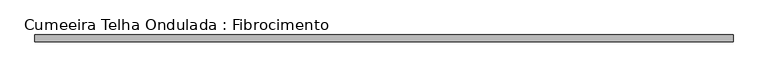
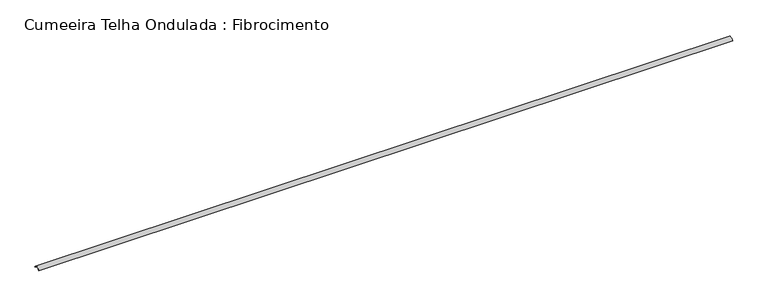
"""IFC4 building model written with IfcOpenShell, lengths in millimetres: beam geometry, Cumeeira Telha Ondulada : Fibrocimento."""

import ifcopenshell
import ifcopenshell.guid

model = None  # the IFC model being written
_history = None  # IfcOwnerHistory: only IFC2X3 demands one
_inside = {}  # id of a spatial element -> (the spatial element, [elements in it])
_under = {}  # id of a project, library or spatial element -> (it, [spatial elements below it])
_declared = {}  # id of a project -> (the project, [libraries it declares])
_typed = {}  # id of a type object -> (the type object, [elements of that type])
_made_of = {}  # id of a material, layer set ... -> (it, [elements and type objects made of it])


def new_model(schema):
    """Start an empty IFC model of exactly this schema.

    Asked for "IFC4X3", IfcOpenShell would pick the latest addendum, in which some entities
    have other attributes; the version numbers below select the first issue.
    IFC2X3 requires an IfcOwnerHistory on every rooted entity: one is made here for all.
    """
    global model, _history
    if schema == "IFC4X3":
        model = ifcopenshell.file(schema_version=(4, 3, 0, 0))
    else:
        model = ifcopenshell.file(schema=schema)
    _inside.clear()
    _under.clear()
    _declared.clear()
    _typed.clear()
    _made_of.clear()
    _history = None
    if model.schema == "IFC2X3":
        org = make("IfcOrganization", Name="unknown")
        user = make(
            "IfcPersonAndOrganization",
            ThePerson=make("IfcPerson", FamilyName="unknown"),
            TheOrganization=org,
        )
        app = make(
            "IfcApplication",
            ApplicationDeveloper=org,
            Version="unknown",
            ApplicationFullName="unknown",
            ApplicationIdentifier="unknown",
        )
        _history = make(
            "IfcOwnerHistory",
            OwningUser=user,
            OwningApplication=app,
            ChangeAction="ADDED",
            CreationDate=0,
        )
    return model


def make(cls, **values):
    """One entity of the class cls with the attributes given. An attribute that is None is left unset."""
    return model.create_entity(
        cls, **{name: value for name, value in values.items() if value is not None}
    )


def rooted(cls, **values):
    """An entity with a GlobalId (a new one), such as an element, a storey or a relation."""
    return make(cls, GlobalId=ifcopenshell.guid.new(), OwnerHistory=_history, **values)


def si_unit(unit_type, name, prefix=None):
    """IfcSIUnit, for example si_unit("LENGTHUNIT", "METRE", prefix="MILLI")."""
    return make("IfcSIUnit", UnitType=unit_type, Prefix=prefix, Name=name)


def assignment(units):
    """IfcUnitAssignment: the units of a project."""
    return None if units is None else make("IfcUnitAssignment", Units=units)


def point(xyz):
    """IfcCartesianPoint."""
    return None if xyz is None else make("IfcCartesianPoint", Coordinates=xyz)


def direction(xyz):
    """IfcDirection."""
    return None if xyz is None else make("IfcDirection", DirectionRatios=xyz)


def frame(location, z_axis=None, x_axis=None):
    """IfcAxis2Placement3D, a coordinate frame: its origin and axes. An axis left out is left unset."""
    return make(
        "IfcAxis2Placement3D",
        Location=point(location),
        Axis=direction(z_axis),
        RefDirection=direction(x_axis),
    )


def frame_2d(location, x_axis=None):
    """IfcAxis2Placement2D, a coordinate frame in the plane: its origin and x axis."""
    return make(
        "IfcAxis2Placement2D", Location=point(location), RefDirection=direction(x_axis)
    )


def origin():
    """The frame at (0, 0, 0) with its axes left unset."""
    return frame((0.0, 0.0, 0.0))


def place(relative_to, where):
    """IfcLocalPlacement: puts the frame where relative to a parent placement (None: the world)."""
    return make(
        "IfcLocalPlacement", PlacementRelTo=relative_to, RelativePlacement=where
    )


def context(
    kind, dimensions, precision=None, world=None, true_north=None, identifier=None
):
    """IfcGeometricRepresentationContext, for example the 3D "Model" context."""
    return make(
        "IfcGeometricRepresentationContext",
        ContextIdentifier=identifier,
        ContextType=kind,
        CoordinateSpaceDimension=dimensions,
        Precision=precision,
        WorldCoordinateSystem=world,
        TrueNorth=true_north,
    )


def project(units=None, contexts=None):
    """IfcProject with its units and contexts."""
    return rooted(
        "IfcProject",
        Name="project",
        RepresentationContexts=contexts,
        UnitsInContext=assignment(units),
    )


def spatial(cls, under=None, at=None, **own):
    """A site, building, storey or space (cls), placed at a placement, below another one or the project."""
    s = rooted(cls, ObjectPlacement=at, **own)
    if under is not None:
        _under.setdefault(under.id(), (under, []))[1].append(s)
    return s


def polyline(points):
    """IfcPolyline through the points."""
    return make("IfcPolyline", Points=[point(p) for p in points])


def circle_curve(where, radius):
    """IfcCircle in the frame where."""
    return make("IfcCircle", Position=where, Radius=radius)


def trimmed(basis, trim1, trim2, sense, master):
    """IfcTrimmedCurve: the piece of a basis curve between two trims."""
    return make(
        "IfcTrimmedCurve",
        BasisCurve=basis,
        Trim1=trim1,
        Trim2=trim2,
        SenseAgreement=sense,
        MasterRepresentation=master,
    )


def segment(curve, same_sense, transition):
    """IfcCompositeCurveSegment."""
    return make(
        "IfcCompositeCurveSegment",
        Transition=transition,
        SameSense=same_sense,
        ParentCurve=curve,
    )


def composite_curve(segments, self_intersect=None):
    """IfcCompositeCurve: segments joined end to end."""
    return make("IfcCompositeCurve", Segments=segments, SelfIntersect=self_intersect)


def outline(outer, holes=None, kind="AREA"):
    """IfcArbitraryClosedProfileDef: a profile drawn as a closed curve; with holes, ...WithVoids."""
    if holes is None:
        return make("IfcArbitraryClosedProfileDef", ProfileType=kind, OuterCurve=outer)
    return make(
        "IfcArbitraryProfileDefWithVoids",
        ProfileType=kind,
        OuterCurve=outer,
        InnerCurves=holes,
    )


def extrude(swept, where, along, depth):
    """IfcExtrudedAreaSolid: the profile swept, set in the frame where, extruded along a direction by depth."""
    return make(
        "IfcExtrudedAreaSolid",
        SweptArea=swept,
        Position=where,
        ExtrudedDirection=direction(along),
        Depth=depth,
    )


def shape(context_of_items, identifier, shape_type, items):
    """IfcShapeRepresentation: the items that make up one representation, for example the "Body"."""
    return make(
        "IfcShapeRepresentation",
        ContextOfItems=context_of_items,
        RepresentationIdentifier=identifier,
        RepresentationType=shape_type,
        Items=items,
    )


def source(mapping_origin, context_of_items, identifier, shape_type, items):
    """IfcRepresentationMap: a shape defined once, which mapped items show again and again."""
    return make(
        "IfcRepresentationMap",
        MappingOrigin=mapping_origin,
        MappedRepresentation=shape(context_of_items, identifier, shape_type, items),
    )


def transform(
    local_origin,
    x_axis=None,
    y_axis=None,
    z_axis=None,
    scale=None,
    scale2=None,
    scale3=None,
    uniform=True,
):
    """IfcCartesianTransformationOperator3D, or its non-uniform kind. x_axis, y_axis, z_axis: its Axis1, 2, 3."""
    if uniform:
        return make(
            "IfcCartesianTransformationOperator3D",
            Axis1=direction(x_axis),
            Axis2=direction(y_axis),
            LocalOrigin=point(local_origin),
            Scale=scale,
            Axis3=direction(z_axis),
        )
    return make(
        "IfcCartesianTransformationOperator3DnonUniform",
        Axis1=direction(x_axis),
        Axis2=direction(y_axis),
        LocalOrigin=point(local_origin),
        Scale=scale,
        Axis3=direction(z_axis),
        Scale2=scale2,
        Scale3=scale3,
    )


def mapped(mapping_source, mapping_target):
    """IfcMappedItem: shows the shape of a source again, moved by a transform."""
    return make(
        "IfcMappedItem", MappingSource=mapping_source, MappingTarget=mapping_target
    )


def made_of(thing, what):
    """Note that an element or type object is made of a material, layer set ...; save() writes the relation."""
    if what is not None:
        _made_of.setdefault(what.id(), (what, []))[1].append(thing)
    return thing


def element(
    cls,
    number,
    at=None,
    inside=None,
    cuts=None,
    type_object=None,
    material=None,
    context=None,
    identifier="Body",
    shape_type=None,
    held_by="IfcProductDefinitionShape",
    body=None,
    shapes=None,
    **own,
):
    """One element of the class cls, such as IfcWall. Its Tag is "e" and its number.

    at: its placement. inside: the storey or other place that contains it. cuts: it is an
    opening in that element (IfcRelVoidsElement). A single representation is given by context,
    identifier, shape_type and body (its items); several are given by shapes. held_by: the class
    of the entity that holds the representations. save() writes the other relations.
    """
    e = rooted(cls, Tag="e%d" % number, ObjectPlacement=at, **own)
    if body is not None:
        shapes = [shape(context, identifier, shape_type, body)]
    if shapes is not None:
        e.Representation = make(held_by, Representations=shapes)
    if inside is not None:
        _inside.setdefault(inside.id(), (inside, []))[1].append(e)
    if cuts is not None:
        rooted(
            "IfcRelVoidsElement", RelatingBuildingElement=cuts, RelatedOpeningElement=e
        )
    if type_object is not None:
        _typed.setdefault(type_object.id(), (type_object, []))[1].append(e)
    return made_of(e, material)


def aggregate(whole, parts):
    """IfcRelAggregates: a whole, such as a stair, and the parts it consists of."""
    return rooted("IfcRelAggregates", RelatingObject=whole, RelatedObjects=parts)


def save(model, path):
    """Write the relations noted so far, then the file.

    IfcRelAggregates (storeys below a building ...), IfcRelContainedInSpatialStructure (elements
    in a storey), IfcRelDefinesByType, IfcRelAssociatesMaterial and IfcRelDeclares: one each for
    every whole, place, type object, material and project.
    """
    for whole, parts in _under.values():
        aggregate(whole, parts)
    for where, things in _inside.values():
        rooted(
            "IfcRelContainedInSpatialStructure",
            RelatedElements=things,
            RelatingStructure=where,
        )
    for kind, things in _typed.values():
        rooted("IfcRelDefinesByType", RelatedObjects=things, RelatingType=kind)
    for what, things in _made_of.values():
        rooted("IfcRelAssociatesMaterial", RelatedObjects=things, RelatingMaterial=what)
    for by, libraries in _declared.values():
        rooted("IfcRelDeclares", RelatingContext=by, RelatedDefinitions=libraries)
    model.write(path)


def cumeeira_telha_ondulada_fibrocimento_4a9e66c1(model_context):
    return source(origin(), model_context, "Body", "SweptSolid", [
        extrude(outline(composite_curve([segment(polyline([(58.3970135, 42.4437972), (53.9055884, 40.2467307)]), True, "CONTINUOUS"), segment(trimmed(circle_curve(frame_2d((-1.6029865, 13.0936483)), 61.7939461), [point((53.9055884, 40.2467307))], [point((-57.1115615, 40.2467307))], True, "CARTESIAN"), True, "CONTINUOUS"), segment(polyline([(-57.1115615, 40.2467307), (-61.6029865, 42.4437972)]), True, "CONTINUOUS"), segment(trimmed(circle_curve(frame_2d((-1.6029865, 13.0936483)), 66.7939461), [point((-61.6029865, 42.4437972))], [point((58.3970135, 42.4437972))], False, "CARTESIAN"), True, "CONTINUOUS")], self_intersect=False)), frame((-6200.0, 0.0, 0.0), z_axis=(1.0, 0.0, 0.0), x_axis=(0.0, 1.0, 0.0)), (0.0, 0.0, 1.0), 12400.0),
    ])


if __name__ == "__main__":
    model = new_model("IFC4")
    model_context = context("Model", 3, world=origin())
    ifc_project = project(units=[si_unit("LENGTHUNIT", "METRE", prefix="MILLI")], contexts=[model_context])
    site = spatial("IfcSite", under=ifc_project)
    building = spatial("IfcBuilding", under=site)
    placement = place(None, origin())
    cumeeira_telha_ondulada_fibrocimento_shape = cumeeira_telha_ondulada_fibrocimento_4a9e66c1(model_context)
    element("IfcBeam", 1, ObjectType="Cumeeira Telha Ondulada : Fibrocimento", at=placement, inside=building, context=model_context, shape_type="MappedRepresentation", body=[
        mapped(cumeeira_telha_ondulada_fibrocimento_shape, transform((0.0, 0.0, 0.0), x_axis=(1.0, 0.0, 0.0), y_axis=(0.0, 1.0, 0.0), z_axis=(0.0, 0.0, 1.0))),
    ])
    save(model, "model.ifc")

# Revit data of these elements
# Type "Cumeeira Telha Ondulada : Fibrocimento"
#   Cost = 5
#   Length [instance default] = 1.524 m
#   b = 0.07 m
#   h = 0.16 m
#   Structural Material = .TELHA DE FIBROCIMENTO
#   Assembly Code = ""
# Element 1 (IfcBeam, "Cumeeira Telha Ondulada : Fibrocimento")
#   Materials on its faces: ".TELHA DE FIBROCIMENTO"
# Materials
#   ".TELHA DE FIBROCIMENTO": class "CC_TELHADO", colour RGB 77 77 76, transparency 0, Description = "TELHA ONDULADA FIBROCIMENTO", Cost = 0
